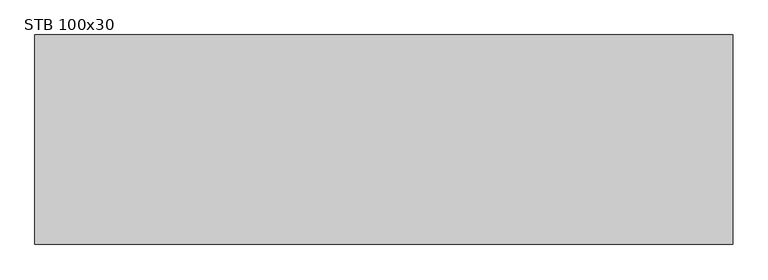
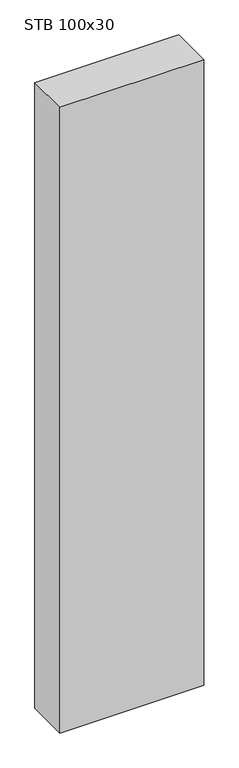
"""IFC4 building model written with IfcOpenShell, lengths in millimetres: column geometry, STB Stütze - rechteckig : STB 100x30."""

from ifc_helpers import new_model, si_unit, frame, origin, place, context, project, spatial, polyline, outline, extrude, source, transform, mapped, element, save


def stb_100x30_1df28cf3(model_context):
    return source(origin(), model_context, "Body", "SweptSolid", [
        extrude(outline(polyline([(500.0, 150.0), (500.0, -150.0), (-500.0, -150.0), (-500.0, 150.0), (500.0, 150.0)])), frame((0.0, 0.0, -1580.0), z_axis=(0.0, 0.0, 1.0), x_axis=(1.0, 0.0, 0.0)), (0.0, 0.0, 1.0), 4600.0),
    ])


if __name__ == "__main__":
    model = new_model("IFC4")
    model_context = context("Model", 3, world=origin())
    ifc_project = project(units=[si_unit("LENGTHUNIT", "METRE", prefix="MILLI")], contexts=[model_context])
    site = spatial("IfcSite", under=ifc_project)
    building = spatial("IfcBuilding", under=site)
    placement = place(None, origin())
    stb_100x30_shape = stb_100x30_1df28cf3(model_context)
    element("IfcColumn", 1, ObjectType="STB Stütze - rechteckig : STB 100x30", at=placement, inside=building, context=model_context, shape_type="MappedRepresentation", body=[
        mapped(stb_100x30_shape, transform((0.0, 0.0, 0.0), x_axis=(1.0, 0.0, 0.0), y_axis=(0.0, 1.0, 0.0), z_axis=(0.0, 0.0, 1.0))),
    ])
    save(model, "model.ifc")

# Revit data of these elements
# Type "STB Stütze - rechteckig : STB 100x30"
#   Breite = 1.000 m
#   Tiefe = 0.300 m
#   Structural Material [instance default] = Stahlbeton - Ortbeton
# Element 1 (IfcColumn, "STB Stütze - rechteckig : STB 100x30")
#   Materials on its faces: "Stahlbeton - Ortbeton"
# Materials
#   "Stahlbeton - Ortbeton": class "Beton", colour RGB 247 247 247, transparency 0, Cost = 0
